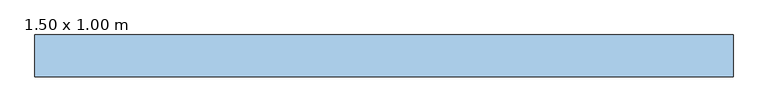
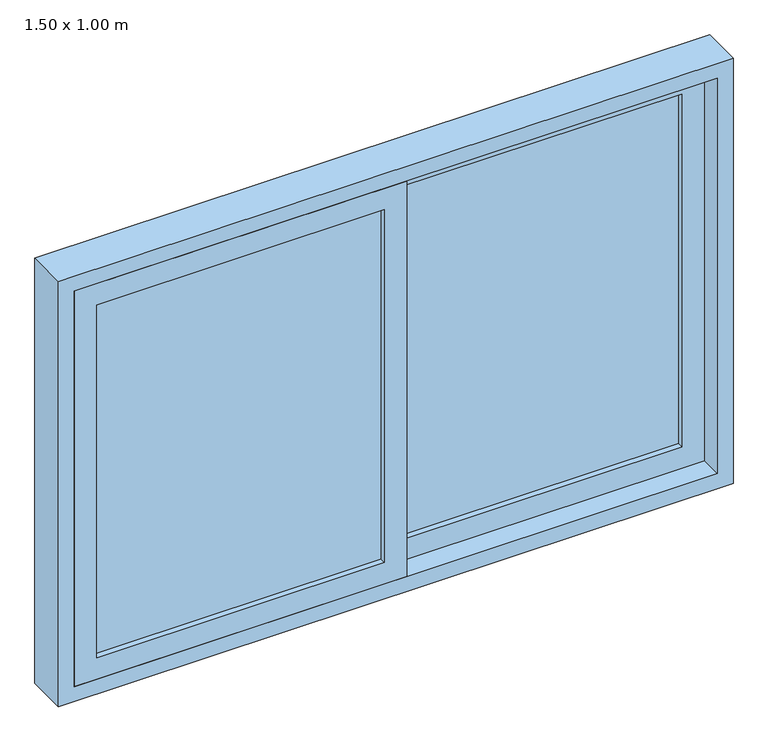
"""IFC4 building model written with IfcOpenShell, lengths in millimetres: window geometry, Janela de correr vidro - 2 Folhas : 1.50 x 1.00 m."""

from ifc_helpers import new_model, si_unit, frame, origin, place, context, project, spatial, polyline, outline, extrude, source, transform, mapped, element, save


def window_1_50_x_1_00_m_3664bad9(model_context):
    return source(origin(), model_context, "Body", "SweptSolid", [
        extrude(outline(polyline([(935.0, -25.0), (935.0, 715.0), (1865.0, 715.0), (1865.0, -25.0), (935.0, -25.0)]), holes=[polyline([(1815.0, 25.0), (1815.0, 665.0), (985.0, 665.0), (985.0, 25.0), (1815.0, 25.0)])]), frame((0.0, -35.0, 0.0), z_axis=(0.0, 1.0, 0.0), x_axis=(0.0, 0.0, 1.0)), (0.0, 0.0, 1.0), 40.0),
        extrude(outline(polyline([(1865.0, 25.0), (1865.0, -715.0), (935.0, -715.0), (935.0, 25.0), (1865.0, 25.0)]), holes=[polyline([(985.0, -25.0), (985.0, -665.0), (1815.0, -665.0), (1815.0, -25.0), (985.0, -25.0)])]), frame((0.0, -85.0, 0.0), z_axis=(0.0, 1.0, 0.0), x_axis=(0.0, 0.0, 1.0)), (0.0, 0.0, 1.0), 40.0),
        extrude(outline(polyline([(1900.0, 750.0), (1900.0, -750.0), (900.0, -750.0), (900.0, 750.0), (1900.0, 750.0)]), holes=[polyline([(935.0, 715.0), (935.0, -715.0), (1865.0, -715.0), (1865.0, 715.0), (935.0, 715.0)])]), frame((0.0, -85.0, 0.0), z_axis=(0.0, 1.0, 0.0), x_axis=(0.0, 0.0, 1.0)), (0.0, 0.0, 1.0), 90.0),
        extrude(outline(polyline([(25.0, -8.0), (665.0, -8.0), (665.0, -22.0), (25.0, -22.0), (25.0, -8.0)])), frame((0.0, 0.0, 985.0), z_axis=(0.0, 0.0, 1.0), x_axis=(1.0, 0.0, 0.0)), (0.0, 0.0, 1.0), 830.0),
        extrude(outline(polyline([(-665.0, -58.0), (-25.0, -58.0), (-25.0, -72.0), (-665.0, -72.0), (-665.0, -58.0)])), frame((0.0, 0.0, 985.0), z_axis=(0.0, 0.0, 1.0), x_axis=(1.0, 0.0, 0.0)), (0.0, 0.0, 1.0), 830.0),
    ])


if __name__ == "__main__":
    model = new_model("IFC4")
    model_context = context("Model", 3, world=origin())
    ifc_project = project(units=[si_unit("LENGTHUNIT", "METRE", prefix="MILLI")], contexts=[model_context])
    site = spatial("IfcSite", under=ifc_project)
    building = spatial("IfcBuilding", under=site)
    placement = place(None, origin())
    window_1_50_x_1_00_m_shape = window_1_50_x_1_00_m_3664bad9(model_context)
    element("IfcWindow", 1, ObjectType="Janela de correr vidro - 2 Folhas : 1.50 x 1.00 m", at=placement, inside=building, context=model_context, shape_type="MappedRepresentation", body=[
        mapped(window_1_50_x_1_00_m_shape, transform((0.0, 0.0, 0.0), x_axis=(1.0, 0.0, 0.0), y_axis=(0.0, 1.0, 0.0), z_axis=(0.0, 0.0, 1.0))),
    ])
    save(model, "model.ifc")

# Revit data of these elements
# Type "Janela de correr vidro - 2 Folhas : 1.50 x 1.00 m"
#   Type Mark = "J17"
#   Construction Type Id = "GSP4R"
#   Analytic Construction = "Vidraça única Pilkington 1/8 pol"
#   Visual Light Transmittance = 0.9
#   Thermal Resistance (R) = 0.271106 (m²·K)/W
#   Solar Heat Gain Coefficient = 0.78
#   Rough Width = 1.500 m
#   Rough Height = 1.000 m
#   Largura da moldura do painel = 0.050 m
#   Espessura da moldura do painel = 0.040 m
#   Height = 1.000 m
#   Heat Transfer Coefficient (U) = 3.6886 W/(m²·K)
#   Largura da estrutura = 0.035 m
#   Espessura da moldura = 0.090 m
#   Altura-padrão do peitoril = 0.900 m
#   Width = 1.500 m
#   Define Thermal Properties by = 1
#   Pingadeira = yes
#   Material da Pingadeira = Granito amarelo
#   Vidro = Vidro
#   Material da estrutura = Metal - Alumínio
#   Wall Closure = (empty or 0)
# Element 1 (IfcWindow, "Janela de correr vidro - 2 Folhas : 1.50 x 1.00 m")
#   Materials on its faces: "Metal - Alumínio", "Vidro"
# Materials
#   "Granito amarelo": class "Genérico", colour RGB 80 80 80, transparency 0, Cost = 0
#   "Vidro": class "Vidro", colour RGB 0 128 192, transparency 0.9
#   "Metal - Alumínio": class "Metal", colour RGB 247 247 247, transparency 0
